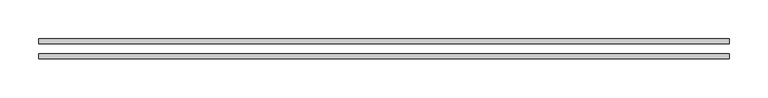
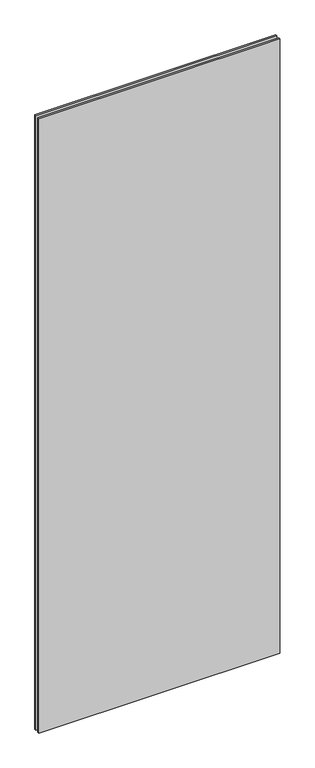
"""IFC4 building model written with IfcOpenShell, lengths in millimetres: proxy geometry, Window glass:Window glass:300352:Window glass:300352 : Window glass:Window glass:300352:300073:Window glass:300352:Window glass:300352 : Window glass:Window glass:300352:300073 : Window glass:Window glass:300352:Window glass:300352 : Window glass:Window glass:300352:300073:1 : Window glass:Window glass:300352:Window glass:300352 : Window glass:Window glass:300352:300073:Window glass:300352:Window glass:300352 : Window glass:Window glass:300352:300073 : Window glass:Window glass:300352:Window glass:300352 : Window glass:Window glass:300352:300073:300061."""

from ifc_helpers import new_model, si_unit, frame, origin, place, context, project, spatial, polyline, outline, extrude, source, transform, mapped, element, save


def generic_models_8e0f790c(model_context):
    return source(origin(), model_context, "Body", "SweptSolid", [
        extrude(outline(polyline([(593690.1661787, -579048.3332724), (592803.3447692, -579048.3332724), (592803.3447692, -579041.9832724), (593690.1661787, -579041.9832724), (593690.1661787, -579048.3332724)])), frame((0.0, 0.0, 55.1405965), z_axis=(0.0, 0.0, 1.0), x_axis=(1.0, 0.0, 0.0)), (0.0, 0.0, 1.0), 2392.531079),
        extrude(outline(polyline([(593690.1661787, -579029.2832724), (592803.3447692, -579029.2832724), (592803.3447692, -579022.9332724), (593690.1661787, -579022.9332724), (593690.1661787, -579029.2832724)])), frame((0.0, 0.0, 55.1405965), z_axis=(0.0, 0.0, 1.0), x_axis=(1.0, 0.0, 0.0)), (0.0, 0.0, 1.0), 2392.531079),
    ])


if __name__ == "__main__":
    model = new_model("IFC4")
    model_context = context("Model", 3, world=origin())
    ifc_project = project(units=[si_unit("LENGTHUNIT", "METRE", prefix="MILLI")], contexts=[model_context])
    site = spatial("IfcSite", under=ifc_project)
    building = spatial("IfcBuilding", under=site)
    placement = place(None, origin())
    generic_models_shape = generic_models_8e0f790c(model_context)
    element("IfcBuildingElementProxy", 1, Name="Window glass:Window glass:300352:Window glass:300352 : Window glass:Window glass:300352:300073:Window glass:300352:Window glass:300352 : Window glass:Window glass:300352:300073 : Window glass:Window glass:300352:Window glass:300352 : Window glass:Window glass:300352:300073:1 : Window glass:Window glass:300352:Window glass:300352 : Window glass:Window glass:300352:300073:Window glass:300352:Window glass:300352 : Window glass:Window glass:300352:300073 : Window glass:Window glass:300352:Window glass:300352 : Window glass:Window glass:300352:300073:300061", ObjectType="Window glass:Window glass:300352:Window glass:300352 : Window glass:Window glass:300352:300073:Window glass:300352:Window glass:300352 : Window glass:Window glass:300352:300073 : Window glass:Window glass:300352:Window glass:300352 : Window glass:Window glass:300352:300073:1 : Window glass:Window glass:300352:Window glass:300352 : Window glass:Window glass:300352:300073:Window glass:300352:Window glass:300352 : Window glass:Window glass:300352:300073 : Window glass:Window glass:300352:Window glass:300352 : Window glass:Window glass:300352:300073:300061", at=placement, inside=building, context=model_context, shape_type="MappedRepresentation", body=[
        mapped(generic_models_shape, transform((0.0, 0.0, 0.0), x_axis=(1.0, 0.0, 0.0), y_axis=(0.0, 1.0, 0.0), z_axis=(0.0, 0.0, 1.0))),
    ])
    save(model, "model.ifc")

# Revit data of these elements
# Type "Window glass:Window glass:300352:Window glass:300352 : Window glass:Window glass:300352:300073:Window glass:300352:Window glass:300352 : Window glass:Window glass:300352:300073 : Window glass:Window glass:300352:Window glass:300352 : Window glass:Window glass:300352:300073:1 : Window glass:Window glass:300352:Window glass:300352 : Window glass:Window glass:300352:300073:Window glass:300352:Window glass:300352 : Window glass:Window glass:300352:300073 : Window glass:Window glass:300352:Window glass:300352 : Window glass:Window glass:300352:300073:300061"
#   NameOverride = "Window glass:Window glass:300352:Window glass:300352 : Window glass:Window glass:300352:300073:Window glass:300352:Window glass:300352 : Window glass:Window glass:300352:300073 : Window glass:Window glass:300352:Window glass:300352 : Window glass:Window glass:300352:300073:300061"
#   ObjectTypeOverride = "Window glass:300352:Window glass:300352 : Window glass:Window glass:300352:300073 : Window glass:Window glass:300352:Window glass:300352 : Window glass:Window glass:300352:300073"
#   Reference = "Window glass"
#   Tag = "300061"
# Element 1 (IfcBuildingElementProxy, "Window glass:Window glass:300352:Window glass:300352 : Window glass:Window glass:300352:300073:Window glass:300352:Window glass:300352 : Window glass:Window glass:300352:300073 : Window glass:Window glass:300352:Window glass:300352 : Window glass:Window glass:300352:300073:1 : Window glass:Window glass:300352:Window glass:300352 : Window glass:Window glass:300352:300073:Window glass:300352:Window glass:300352 : Window glass:Window glass:300352:300073 : Window glass:Window glass:300352:Window glass:300352 : Window glass:Window glass:300352:300073:300061")
#   Materials on its faces: "INSULATED LOW-E GLAZING (SEE ELEVATIONS FOR U-FACTOR, SHGC, & LT)"
# Materials
#   "INSULATED LOW-E GLAZING (SEE ELEVATIONS FOR U-FACTOR, SHGC, & LT)": class "Unassigned", colour RGB 84 171 255, transparency 0, Cost = 0
